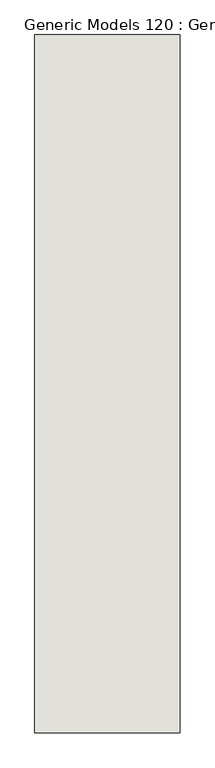
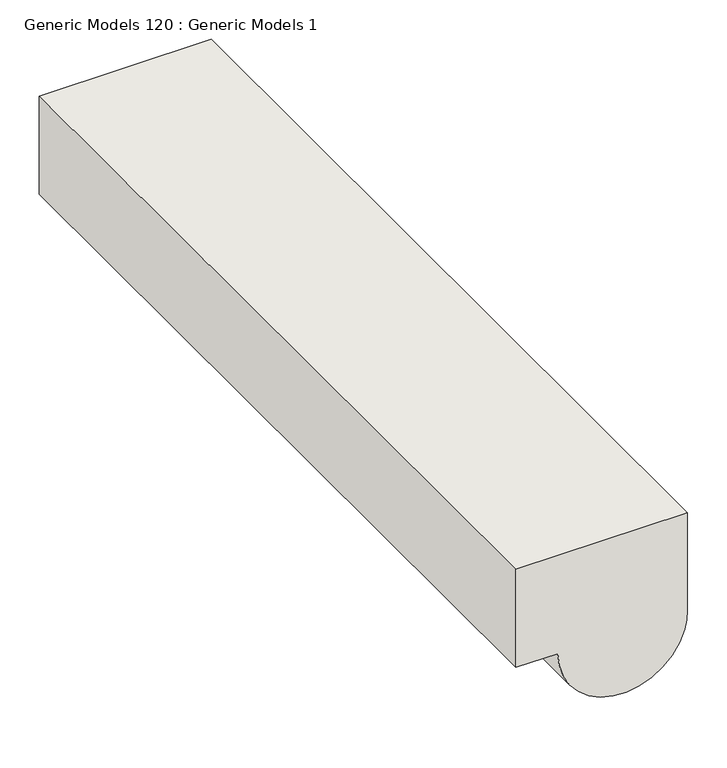
"""IFC4 building model written with IfcOpenShell, lengths in millimetres: wall geometry, Generic Models 120 : Generic Models 1."""

from ifc_helpers import new_model, si_unit, point, frame, frame_2d, origin, place, context, project, spatial, polyline, circle_curve, trimmed, segment, composite_curve, outline, extrude, source, transform, mapped, element, save


def generic_models_120_generic_models_1_590b71c7(model_context):
    return source(origin(), model_context, "Body", "SweptSolid", [
        extrude(outline(composite_curve([segment(polyline([(2540.0, 373859.425), (2540.0, 373607.0125), (2387.5999999, 373607.0125), (2387.5999999, 373668.925)]), True, "CONTINUOUS"), segment(trimmed(circle_curve(frame_2d((2387.5999999, 373764.175)), 95.25), [point((2387.5999999, 373668.925))], [point((2360.0836351, 373855.3638818))], False, "CARTESIAN"), True, "CONTINUOUS"), segment(trimmed(circle_curve(frame_2d((2387.5999999, 373764.175)), 95.25), [point((2360.0836351, 373855.3638818))], [point((2387.5999999, 373859.425))], False, "CARTESIAN"), True, "CONTINUOUS"), segment(polyline([(2387.5999999, 373859.425), (2540.0, 373859.425)]), True, "CONTINUOUS")], self_intersect=False)), frame((0.0, -686.1747735, 0.0), z_axis=(0.0, 1.0, 0.0), x_axis=(0.0, 0.0, 1.0)), (0.0, 0.0, 1.0), 1212.3817147),
    ])


if __name__ == "__main__":
    model = new_model("IFC4")
    model_context = context("Model", 3, world=origin())
    ifc_project = project(units=[si_unit("LENGTHUNIT", "METRE", prefix="MILLI")], contexts=[model_context])
    site = spatial("IfcSite", under=ifc_project)
    building = spatial("IfcBuilding", under=site)
    placement = place(None, origin())
    generic_models_120_generic_models_1_shape = generic_models_120_generic_models_1_590b71c7(model_context)
    element("IfcWall", 1, ObjectType="Generic Models 120 : Generic Models 1", at=placement, inside=building, context=model_context, shape_type="MappedRepresentation", body=[
        mapped(generic_models_120_generic_models_1_shape, transform((0.0, 0.0, 0.0), x_axis=(1.0, 0.0, 0.0), y_axis=(0.0, 1.0, 0.0), z_axis=(0.0, 0.0, 1.0))),
    ])
    save(model, "model.ifc")

# Revit data of these elements
# Element 1 (IfcWall, "Generic Models 120 : Generic Models 1")
#   Materials on its faces: "REINFORCEMENT GROUTED INTO BROKEN CORE"
# Materials
#   "REINFORCEMENT GROUTED INTO BROKEN CORE": class "Generic", colour RGB 255 255 255, transparency 0, Description = "Gypsum Wall Board", Cost = 0
